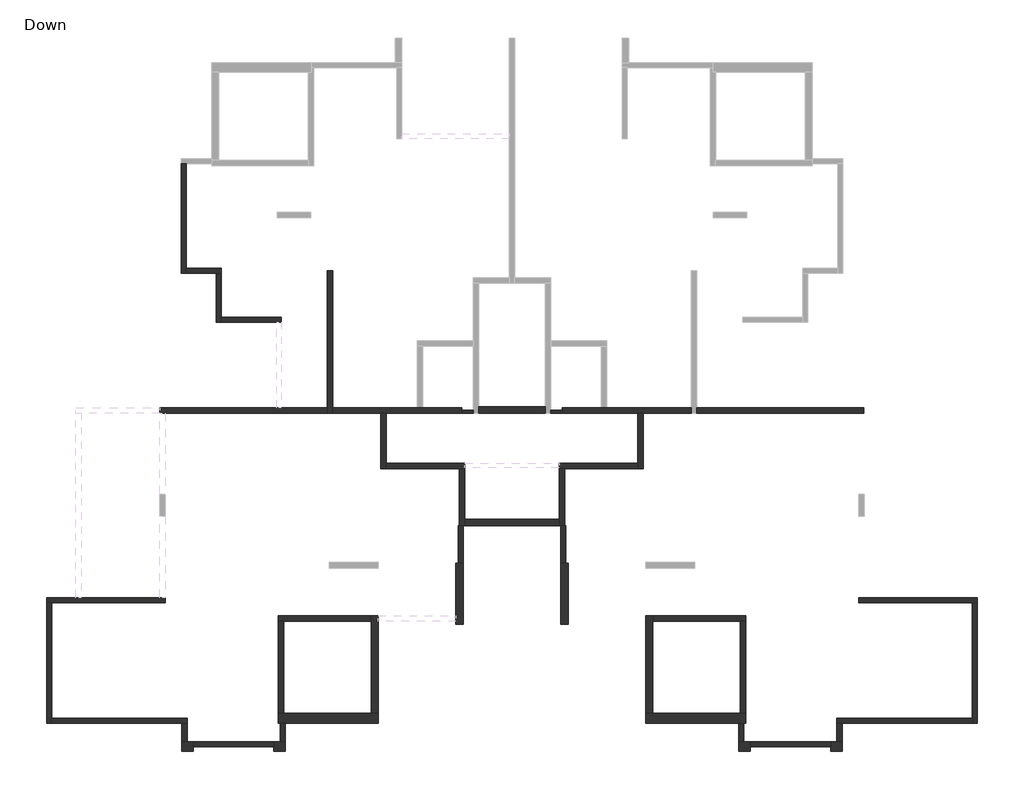
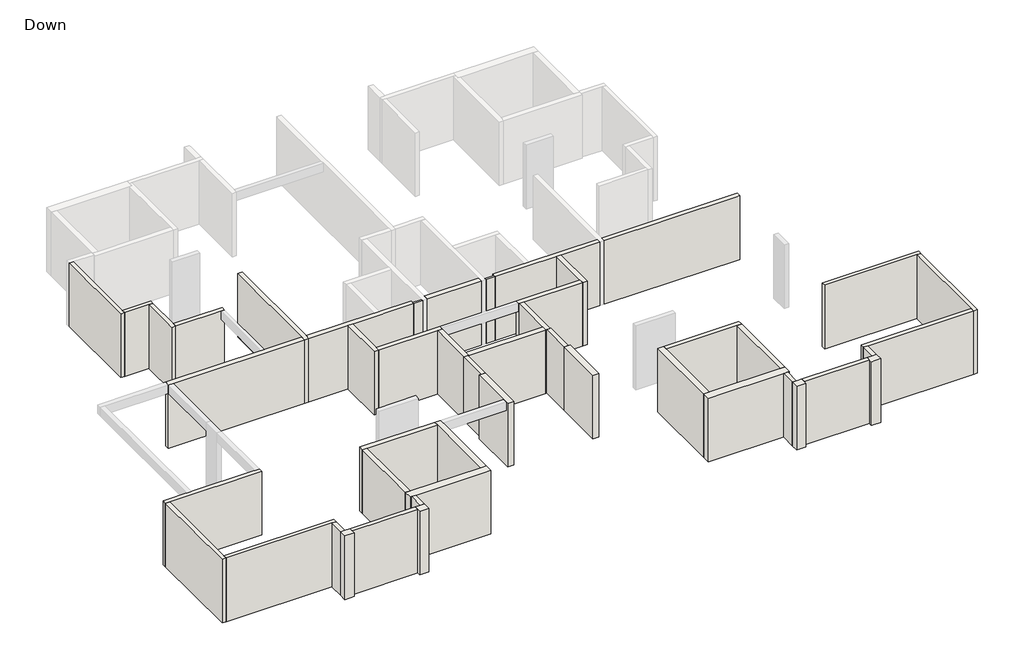
# One storey, part 1 of 2: 47 walls.
# Revit data of these elements (continued)
# Element 24 (IfcWall, "20") (continued)
#   SOFiSTiK_EdgeZones = "W42"
#   SOFiSTiK_AMG_Comments = ""
#   Top Offset = 0 cm
#   Base Offset = 0 cm
#   wall height = 297 cm
#   SOFiSTiK_AMG_Scheduled = yes
#   SOFiSTiK_AMG_Adjusted = yes
#   Phase Created = New Construction
#   Base Constraint = Down
#   Top Constraint = Typical Floor
#   Materials on its faces: "Concrete"
# Element 25 (IfcWall, "20")
#   Comments = ""
#   Mark = "W48"
#   SOFiSTiK_EdgeZones = "W48"
#   SOFiSTiK_AMG_Comments = ""
#   Top Offset = 0 cm
#   Base Offset = 0 cm
#   wall height = 297 cm
#   SOFiSTiK_AMG_Scheduled = yes
#   SOFiSTiK_AMG_Adjusted = yes
#   Phase Created = New Construction
#   Base Constraint = Down
#   Top Constraint = Typical Floor
#   Materials on its faces: "Concrete"
# Element 26 (IfcWall, "20")
#   Comments = ""
#   Mark = "W49"
#   SOFiSTiK_EdgeZones = "W49"
#   SOFiSTiK_AMG_Comments = ""
#   Top Offset = 0 cm
#   Base Offset = 0 cm
#   wall height = 297 cm
#   SOFiSTiK_AMG_Scheduled = yes
#   SOFiSTiK_AMG_Adjusted = yes
#   Phase Created = New Construction
#   Base Constraint = Down
#   Top Constraint = Typical Floor
#   Materials on its faces: "Concrete"
# Element 27 (IfcWall, "20")
#   Comments = ""
#   Mark = "W50"
#   SOFiSTiK_EdgeZones = "W50"
#   SOFiSTiK_AMG_Comments = ""
#   Top Offset = 0 cm
#   Base Offset = 0 cm
#   wall height = 297 cm
#   SOFiSTiK_AMG_Scheduled = yes
#   SOFiSTiK_AMG_Adjusted = yes
#   Phase Created = New Construction
#   Base Constraint = Down
#   Top Constraint = Typical Floor
#   Materials on its faces: "Concrete"
# Element 28 (IfcWall, "20")
#   Comments = ""
#   Mark = "W51"
#   SOFiSTiK_EdgeZones = "W51"
#   SOFiSTiK_AMG_Comments = ""
#   Top Offset = 0 cm
#   Base Offset = 0 cm
#   wall height = 297 cm
#   SOFiSTiK_AMG_Scheduled = yes
#   SOFiSTiK_AMG_Adjusted = yes
#   Phase Created = New Construction
#   Base Constraint = Down
#   Top Constraint = Typical Floor
#   Materials on its faces: "Concrete"
# Element 29 (IfcWall, "20")
#   Comments = ""
#   Mark = "W55"
#   SOFiSTiK_EdgeZones = "W55"
#   SOFiSTiK_AMG_Comments = ""
#   Top Offset = 0 cm
#   Base Offset = 0 cm
#   wall height = 297 cm
#   SOFiSTiK_AMG_Scheduled = yes
#   SOFiSTiK_AMG_Adjusted = yes
#   Phase Created = New Construction
#   Base Constraint = Down
#   Top Constraint = Typical Floor
#   Materials on its faces: "Concrete"
# Element 30 (IfcWall, "20")
#   Comments = ""
#   Mark = "W56"
#   SOFiSTiK_EdgeZones = "W56"
#   SOFiSTiK_AMG_Comments = ""
#   Top Offset = 0 cm
#   Base Offset = 0 cm
#   wall height = 297 cm
#   SOFiSTiK_AMG_Scheduled = yes
#   SOFiSTiK_AMG_Adjusted = yes
#   Phase Created = New Construction
#   Base Constraint = Down
#   Top Constraint = Typical Floor
#   Materials on its faces: "Concrete"
# Element 31 (IfcWall, "20")
#   Comments = ""
#   Mark = "W57"
#   SOFiSTiK_EdgeZones = "W57"
#   SOFiSTiK_AMG_Comments = ""
#   Top Offset = 0 cm
#   Base Offset = 0 cm
#   wall height = 297 cm
#   SOFiSTiK_AMG_Scheduled = yes
#   SOFiSTiK_AMG_Adjusted = yes
#   Phase Created = New Construction
#   Base Constraint = Down
#   Top Constraint = Typical Floor
#   Materials on its faces: "Concrete"
# Element 32 (IfcWall, "20")
#   Comments = ""
#   Mark = "W62"
#   SOFiSTiK_EdgeZones = "W62"
#   SOFiSTiK_AMG_Comments = ""
#   Top Offset = 0 cm
#   Base Offset = 0 cm
#   wall height = 297 cm
#   SOFiSTiK_AMG_Scheduled = yes
#   SOFiSTiK_AMG_Adjusted = yes
#   Phase Created = New Construction
#   Base Constraint = Down
#   Top Constraint = Typical Floor
#   Materials on its faces: "Concrete"
# Element 33 (IfcWall, "20")
#   Comments = ""
#   Mark = "W63"
#   SOFiSTiK_EdgeZones = "W63"
#   SOFiSTiK_AMG_Comments = ""
#   Top Offset = 0 cm
#   Base Offset = 0 cm
#   wall height = 297 cm
#   SOFiSTiK_AMG_Scheduled = yes
#   SOFiSTiK_AMG_Adjusted = yes
#   Phase Created = New Construction
#   Base Constraint = Down
#   Top Constraint = Typical Floor
#   Materials on its faces: "Concrete"
# Element 34 (IfcWall, "20")
#   Comments = ""
#   Mark = "W64"
#   SOFiSTiK_EdgeZones = "W64"
#   SOFiSTiK_AMG_Comments = ""
#   Top Offset = 0 cm
#   Base Offset = 0 cm
#   wall height = 297 cm
#   SOFiSTiK_AMG_Scheduled = yes
#   SOFiSTiK_AMG_Adjusted = yes
#   Phase Created = New Construction
#   Base Constraint = Down
#   Top Constraint = Typical Floor
#   Materials on its faces: "Concrete"
# Element 35 (IfcWall, "20")
#   Comments = ""
#   Mark = "W65"
#   SOFiSTiK_EdgeZones = "W65"
#   SOFiSTiK_AMG_Comments = ""
#   Top Offset = 0 cm
#   Base Offset = 0 cm
#   wall height = 297 cm
#   SOFiSTiK_AMG_Scheduled = yes
#   SOFiSTiK_AMG_Adjusted = yes
#   Phase Created = New Construction
#   Base Constraint = Down
#   Top Constraint = Typical Floor
#   Materials on its faces: "Concrete"
# Element 36 (IfcWall, "23")
#   Comments = ""
#   Mark = "W34"
#   SOFiSTiK_EdgeZones = "W34"
#   SOFiSTiK_AMG_Comments = ""
#   Top Offset = 0 cm
#   Base Offset = 0 cm
#   wall height = 297 cm
#   SOFiSTiK_AMG_Scheduled = yes
#   SOFiSTiK_AMG_Adjusted = yes
#   Phase Created = New Construction
#   Base Constraint = Down
#   Top Constraint = Typical Floor
#   Materials on its faces: "Concrete"
# Element 37 (IfcWall, "23")
#   Comments = ""
#   Mark = "W36"
#   SOFiSTiK_EdgeZones = "W36"
#   SOFiSTiK_AMG_Comments = ""
#   Top Offset = 0 cm
#   Base Offset = 0 cm
#   wall height = 297 cm
#   SOFiSTiK_AMG_Scheduled = yes
#   SOFiSTiK_AMG_Adjusted = yes
#   Phase Created = New Construction
#   Base Constraint = Down
#   Top Constraint = Typical Floor
#   Materials on its faces: "Concrete"
# Element 38 (IfcWall, "25")
#   Comments = ""
#   Mark = "W67"
#   SOFiSTiK_EdgeZones = "W67"
#   SOFiSTiK_AMG_Comments = ""
#   Top Offset = 0 cm
#   Base Offset = 0 cm
#   wall height = 297 cm
#   SOFiSTiK_AMG_Scheduled = yes
#   SOFiSTiK_AMG_Adjusted = yes
#   Phase Created = New Construction
#   Base Constraint = Down
#   Top Constraint = Typical Floor
#   Materials on its faces: "Concrete"
# Element 39 (IfcWall, "25")
#   Comments = ""
#   Mark = "W69"
#   SOFiSTiK_EdgeZones = "W69"
#   SOFiSTiK_AMG_Comments = ""
#   Top Offset = 0 cm
#   Base Offset = 0 cm
#   wall height = 297 cm
#   SOFiSTiK_AMG_Scheduled = yes
#   SOFiSTiK_AMG_Adjusted = yes
#   Phase Created = New Construction
#   Base Constraint = Down
#   Top Constraint = Typical Floor
#   Materials on its faces: "Concrete"
# Element 40 (IfcWall, "27")
#   Comments = ""
#   Mark = "W76"
#   SOFiSTiK_EdgeZones = "W76"
#   SOFiSTiK_AMG_Comments = ""
#   Top Offset = 0 cm
#   Base Offset = 0 cm
#   wall height = 297 cm
#   SOFiSTiK_AMG_Scheduled = yes
#   SOFiSTiK_AMG_Adjusted = yes
#   Phase Created = New Construction
#   Base Constraint = Down
#   Top Constraint = Typical Floor
#   Materials on its faces: "Concrete"
# Element 41 (IfcWall, "27")
#   Comments = ""
#   Mark = "W77"
#   SOFiSTiK_EdgeZones = "W77"
#   SOFiSTiK_AMG_Comments = ""
#   Top Offset = 0 cm
#   Base Offset = 0 cm
#   wall height = 297 cm
#   SOFiSTiK_AMG_Scheduled = yes
#   SOFiSTiK_AMG_Adjusted = yes
#   Phase Created = New Construction
#   Base Constraint = Down
#   Top Constraint = Typical Floor
#   Materials on its faces: "Concrete"
# Element 42 (IfcWall, "33")
#   Comments = ""
#   Mark = "W70"
#   SOFiSTiK_EdgeZones = "W70"
#   SOFiSTiK_AMG_Comments = ""
#   Top Offset = 0 cm
#   Base Offset = 0 cm
#   wall height = 297 cm
#   SOFiSTiK_AMG_Scheduled = yes
#   SOFiSTiK_AMG_Adjusted = yes
#   Phase Created = New Construction
#   Base Constraint = Down
#   Top Constraint = Typical Floor
#   Materials on its faces: "Concrete"
# Element 43 (IfcWall, "33")
#   Comments = ""
#   Mark = "W71"
#   SOFiSTiK_EdgeZones = "W71"
#   SOFiSTiK_AMG_Comments = ""
#   Top Offset = 0 cm
#   Base Offset = 0 cm
#   wall height = 297 cm
#   SOFiSTiK_AMG_Scheduled = yes
#   SOFiSTiK_AMG_Adjusted = yes
#   Phase Created = New Construction
#   Base Constraint = Down
#   Top Constraint = Typical Floor
#   Materials on its faces: "Concrete"
# Element 44 (IfcWall, "33")
#   Comments = ""
#   Mark = "W72"
#   SOFiSTiK_EdgeZones = "W72"
#   SOFiSTiK_AMG_Comments = ""
#   Top Offset = 0 cm
#   Base Offset = 0 cm
#   wall height = 297 cm
#   SOFiSTiK_AMG_Scheduled = yes
#   SOFiSTiK_AMG_Adjusted = yes
#   Phase Created = New Construction
#   Base Constraint = Down
#   Top Constraint = Typical Floor
#   Materials on its faces: "Concrete"
# Element 45 (IfcWall, "33")
#   Comments = ""
#   Mark = "W73"
#   SOFiSTiK_EdgeZones = "W73"
#   SOFiSTiK_AMG_Comments = ""
#   Top Offset = 0 cm
#   Base Offset = 0 cm
#   wall height = 297 cm
#   SOFiSTiK_AMG_Scheduled = yes
#   SOFiSTiK_AMG_Adjusted = yes
#   Phase Created = New Construction
#   Base Constraint = Down
#   Top Constraint = Typical Floor
#   Materials on its faces: "Concrete"
# Element 46 (IfcWall, "35")
#   Comments = ""
#   Mark = "W2"
#   SOFiSTiK_EdgeZones = "W2"
#   SOFiSTiK_AMG_Comments = ""
#   Top Offset = 0 cm
#   Base Offset = 0 cm
#   wall height = 297 cm
#   SOFiSTiK_AMG_Scheduled = yes
#   SOFiSTiK_AMG_Adjusted = yes
#   Phase Created = New Construction
#   Base Constraint = Down
#   Top Constraint = Typical Floor
#   Materials on its faces: "Concrete"
# Element 47 (IfcWall, "35")
#   Comments = ""
#   Mark = "W4"
#   SOFiSTiK_EdgeZones = "W4"
#   SOFiSTiK_AMG_Comments = ""
#   Top Offset = 0 cm
#   Base Offset = 0 cm
#   wall height = 297 cm
#   SOFiSTiK_AMG_Scheduled = yes
#   SOFiSTiK_AMG_Adjusted = yes
#   Phase Created = New Construction
#   Base Constraint = Down
#   Top Constraint = Typical Floor
#   Materials on its faces: "Concrete"
# Materials
#   "Concrete": class "Concrete", colour RGB 192 192 192, transparency 0, Keynote = "01000", Description = "Cast-in-place concrete", Cost = 0
